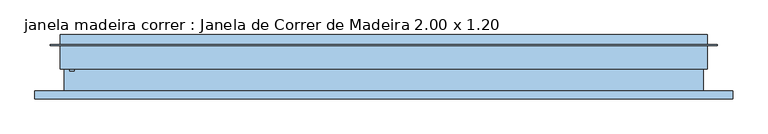
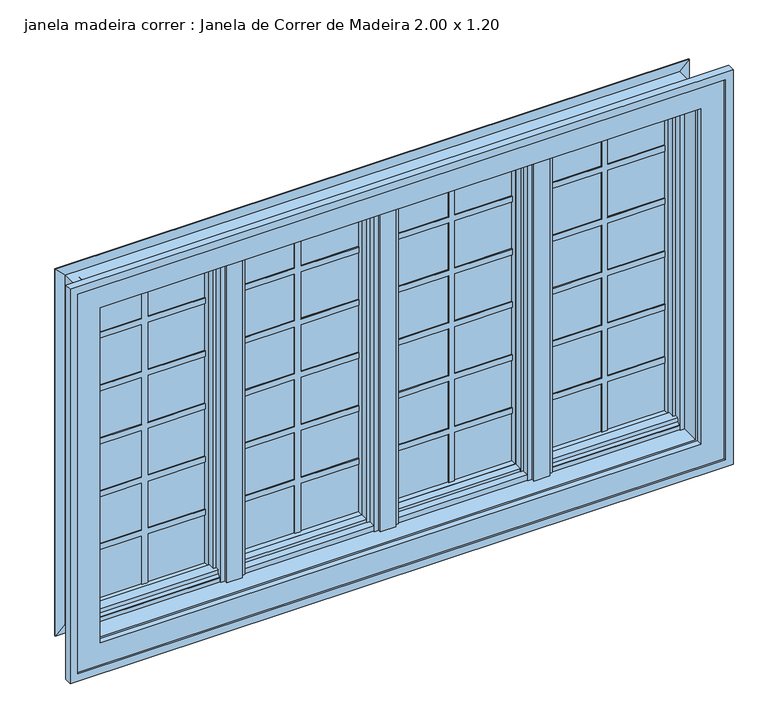
"""IFC4 building model written with IfcOpenShell, lengths in millimetres: window geometry, janela madeira correr : Janela de Correr de Madeira 2.00 x 1.20."""

import ifcopenshell
import ifcopenshell.guid

model = None  # the IFC model being written
_history = None  # IfcOwnerHistory: only IFC2X3 demands one
_inside = {}  # id of a spatial element -> (the spatial element, [elements in it])
_under = {}  # id of a project, library or spatial element -> (it, [spatial elements below it])
_declared = {}  # id of a project -> (the project, [libraries it declares])
_typed = {}  # id of a type object -> (the type object, [elements of that type])
_made_of = {}  # id of a material, layer set ... -> (it, [elements and type objects made of it])


def new_model(schema):
    """Start an empty IFC model of exactly this schema.

    Asked for "IFC4X3", IfcOpenShell would pick the latest addendum, in which some entities
    have other attributes; the version numbers below select the first issue.
    IFC2X3 requires an IfcOwnerHistory on every rooted entity: one is made here for all.
    """
    global model, _history
    if schema == "IFC4X3":
        model = ifcopenshell.file(schema_version=(4, 3, 0, 0))
    else:
        model = ifcopenshell.file(schema=schema)
    _inside.clear()
    _under.clear()
    _declared.clear()
    _typed.clear()
    _made_of.clear()
    _history = None
    if model.schema == "IFC2X3":
        org = make("IfcOrganization", Name="unknown")
        user = make(
            "IfcPersonAndOrganization",
            ThePerson=make("IfcPerson", FamilyName="unknown"),
            TheOrganization=org,
        )
        app = make(
            "IfcApplication",
            ApplicationDeveloper=org,
            Version="unknown",
            ApplicationFullName="unknown",
            ApplicationIdentifier="unknown",
        )
        _history = make(
            "IfcOwnerHistory",
            OwningUser=user,
            OwningApplication=app,
            ChangeAction="ADDED",
            CreationDate=0,
        )
    return model


def make(cls, **values):
    """One entity of the class cls with the attributes given. An attribute that is None is left unset."""
    return model.create_entity(
        cls, **{name: value for name, value in values.items() if value is not None}
    )


def rooted(cls, **values):
    """An entity with a GlobalId (a new one), such as an element, a storey or a relation."""
    return make(cls, GlobalId=ifcopenshell.guid.new(), OwnerHistory=_history, **values)


def si_unit(unit_type, name, prefix=None):
    """IfcSIUnit, for example si_unit("LENGTHUNIT", "METRE", prefix="MILLI")."""
    return make("IfcSIUnit", UnitType=unit_type, Prefix=prefix, Name=name)


def assignment(units):
    """IfcUnitAssignment: the units of a project."""
    return None if units is None else make("IfcUnitAssignment", Units=units)


def point(xyz):
    """IfcCartesianPoint."""
    return None if xyz is None else make("IfcCartesianPoint", Coordinates=xyz)


def direction(xyz):
    """IfcDirection."""
    return None if xyz is None else make("IfcDirection", DirectionRatios=xyz)


def frame(location, z_axis=None, x_axis=None):
    """IfcAxis2Placement3D, a coordinate frame: its origin and axes. An axis left out is left unset."""
    return make(
        "IfcAxis2Placement3D",
        Location=point(location),
        Axis=direction(z_axis),
        RefDirection=direction(x_axis),
    )


def origin():
    """The frame at (0, 0, 0) with its axes left unset."""
    return frame((0.0, 0.0, 0.0))


def place(relative_to, where):
    """IfcLocalPlacement: puts the frame where relative to a parent placement (None: the world)."""
    return make(
        "IfcLocalPlacement", PlacementRelTo=relative_to, RelativePlacement=where
    )


def context(
    kind, dimensions, precision=None, world=None, true_north=None, identifier=None
):
    """IfcGeometricRepresentationContext, for example the 3D "Model" context."""
    return make(
        "IfcGeometricRepresentationContext",
        ContextIdentifier=identifier,
        ContextType=kind,
        CoordinateSpaceDimension=dimensions,
        Precision=precision,
        WorldCoordinateSystem=world,
        TrueNorth=true_north,
    )


def project(units=None, contexts=None):
    """IfcProject with its units and contexts."""
    return rooted(
        "IfcProject",
        Name="project",
        RepresentationContexts=contexts,
        UnitsInContext=assignment(units),
    )


def spatial(cls, under=None, at=None, **own):
    """A site, building, storey or space (cls), placed at a placement, below another one or the project."""
    s = rooted(cls, ObjectPlacement=at, **own)
    if under is not None:
        _under.setdefault(under.id(), (under, []))[1].append(s)
    return s


def polyline(points):
    """IfcPolyline through the points."""
    return make("IfcPolyline", Points=[point(p) for p in points])


def outline(outer, holes=None, kind="AREA"):
    """IfcArbitraryClosedProfileDef: a profile drawn as a closed curve; with holes, ...WithVoids."""
    if holes is None:
        return make("IfcArbitraryClosedProfileDef", ProfileType=kind, OuterCurve=outer)
    return make(
        "IfcArbitraryProfileDefWithVoids",
        ProfileType=kind,
        OuterCurve=outer,
        InnerCurves=holes,
    )


def extrude(swept, where, along, depth):
    """IfcExtrudedAreaSolid: the profile swept, set in the frame where, extruded along a direction by depth."""
    return make(
        "IfcExtrudedAreaSolid",
        SweptArea=swept,
        Position=where,
        ExtrudedDirection=direction(along),
        Depth=depth,
    )


def faces_of(points, faces, orient=None, outer=None):
    """IfcFace entities. A face is a list of loops; a loop is a list of indices into points, from 0.

    orient and outer hold one flag for each loop. By default every Orientation is true, the
    first loop of a face is its IfcFaceOuterBound and the others are IfcFaceBound.
    """
    made = []
    for i, loops in enumerate(faces):
        bounds = []
        for j, loop in enumerate(loops):
            is_outer = j == 0 if outer is None else outer[i][j]
            bounds.append(
                make(
                    "IfcFaceOuterBound" if is_outer else "IfcFaceBound",
                    Bound=make("IfcPolyLoop", Polygon=[points[k] for k in loop]),
                    Orientation=True if orient is None else orient[i][j],
                )
            )
        made.append(make("IfcFace", Bounds=bounds))
    return made


def faceted_brep(points, faces, orient=None, outer=None, voids=None):
    """IfcFacetedBrep: a solid bounded by flat faces; with voids (closed shells), ...WithVoids."""
    shared = [point(p) for p in points]
    hull = make("IfcClosedShell", CfsFaces=faces_of(shared, faces, orient, outer))
    if voids is None:
        return make("IfcFacetedBrep", Outer=hull)
    return make(
        "IfcFacetedBrepWithVoids",
        Outer=hull,
        Voids=[
            make(cls, CfsFaces=faces_of(shared, fs, o, b)) for cls, fs, o, b in voids
        ],
    )


def shape(context_of_items, identifier, shape_type, items):
    """IfcShapeRepresentation: the items that make up one representation, for example the "Body"."""
    return make(
        "IfcShapeRepresentation",
        ContextOfItems=context_of_items,
        RepresentationIdentifier=identifier,
        RepresentationType=shape_type,
        Items=items,
    )


def source(mapping_origin, context_of_items, identifier, shape_type, items):
    """IfcRepresentationMap: a shape defined once, which mapped items show again and again."""
    return make(
        "IfcRepresentationMap",
        MappingOrigin=mapping_origin,
        MappedRepresentation=shape(context_of_items, identifier, shape_type, items),
    )


def transform(
    local_origin,
    x_axis=None,
    y_axis=None,
    z_axis=None,
    scale=None,
    scale2=None,
    scale3=None,
    uniform=True,
):
    """IfcCartesianTransformationOperator3D, or its non-uniform kind. x_axis, y_axis, z_axis: its Axis1, 2, 3."""
    if uniform:
        return make(
            "IfcCartesianTransformationOperator3D",
            Axis1=direction(x_axis),
            Axis2=direction(y_axis),
            LocalOrigin=point(local_origin),
            Scale=scale,
            Axis3=direction(z_axis),
        )
    return make(
        "IfcCartesianTransformationOperator3DnonUniform",
        Axis1=direction(x_axis),
        Axis2=direction(y_axis),
        LocalOrigin=point(local_origin),
        Scale=scale,
        Axis3=direction(z_axis),
        Scale2=scale2,
        Scale3=scale3,
    )


def mapped(mapping_source, mapping_target):
    """IfcMappedItem: shows the shape of a source again, moved by a transform."""
    return make(
        "IfcMappedItem", MappingSource=mapping_source, MappingTarget=mapping_target
    )


def made_of(thing, what):
    """Note that an element or type object is made of a material, layer set ...; save() writes the relation."""
    if what is not None:
        _made_of.setdefault(what.id(), (what, []))[1].append(thing)
    return thing


def element(
    cls,
    number,
    at=None,
    inside=None,
    cuts=None,
    type_object=None,
    material=None,
    context=None,
    identifier="Body",
    shape_type=None,
    held_by="IfcProductDefinitionShape",
    body=None,
    shapes=None,
    **own,
):
    """One element of the class cls, such as IfcWall. Its Tag is "e" and its number.

    at: its placement. inside: the storey or other place that contains it. cuts: it is an
    opening in that element (IfcRelVoidsElement). A single representation is given by context,
    identifier, shape_type and body (its items); several are given by shapes. held_by: the class
    of the entity that holds the representations. save() writes the other relations.
    """
    e = rooted(cls, Tag="e%d" % number, ObjectPlacement=at, **own)
    if body is not None:
        shapes = [shape(context, identifier, shape_type, body)]
    if shapes is not None:
        e.Representation = make(held_by, Representations=shapes)
    if inside is not None:
        _inside.setdefault(inside.id(), (inside, []))[1].append(e)
    if cuts is not None:
        rooted(
            "IfcRelVoidsElement", RelatingBuildingElement=cuts, RelatedOpeningElement=e
        )
    if type_object is not None:
        _typed.setdefault(type_object.id(), (type_object, []))[1].append(e)
    return made_of(e, material)


def aggregate(whole, parts):
    """IfcRelAggregates: a whole, such as a stair, and the parts it consists of."""
    return rooted("IfcRelAggregates", RelatingObject=whole, RelatedObjects=parts)


def save(model, path):
    """Write the relations noted so far, then the file.

    IfcRelAggregates (storeys below a building ...), IfcRelContainedInSpatialStructure (elements
    in a storey), IfcRelDefinesByType, IfcRelAssociatesMaterial and IfcRelDeclares: one each for
    every whole, place, type object, material and project.
    """
    for whole, parts in _under.values():
        aggregate(whole, parts)
    for where, things in _inside.values():
        rooted(
            "IfcRelContainedInSpatialStructure",
            RelatedElements=things,
            RelatingStructure=where,
        )
    for kind, things in _typed.values():
        rooted("IfcRelDefinesByType", RelatedObjects=things, RelatingType=kind)
    for what, things in _made_of.values():
        rooted("IfcRelAssociatesMaterial", RelatedObjects=things, RelatingMaterial=what)
    for by, libraries in _declared.values():
        rooted("IfcRelDeclares", RelatingContext=by, RelatedDefinitions=libraries)
    model.write(path)


def janela_madeira_correr_janela_de_correr_de_madeira_2_00_x_1_d447c460(model_context):
    return source(origin(), model_context, "Body", "SolidModel", [
        extrude(outline(polyline([(1881.6300584, 206.5264803), (1881.6300584, 13.2337398), (1862.5800584, 13.2337398), (1862.5800584, 206.5264803), (1699.6775292, 206.5264803), (1699.6775292, 13.2337398), (1680.6275292, 13.2337398), (1680.6275292, 206.5264803), (1517.725, 206.5264803), (1517.725, 13.2337398), (1498.675, 13.2337398), (1498.675, 206.5264803), (1335.7724708, 206.5264803), (1335.7724708, 13.2337398), (1316.7224708, 13.2337398), (1316.7224708, 206.5264803), (1153.8199416, 206.5264803), (1153.8199416, 13.2337398), (1134.7699416, 13.2337398), (1134.7699416, 206.5264803), (962.3424123, 206.5264803), (962.3424123, 225.5764803), (1134.7699416, 225.5764803), (1134.7699416, 418.8692207), (1153.8199416, 418.8692207), (1153.8199416, 225.5764803), (1316.7224708, 225.5764803), (1316.7224708, 418.8692207), (1335.7724708, 418.8692207), (1335.7724708, 225.5764803), (1498.675, 225.5764803), (1498.675, 418.8692207), (1517.725, 418.8692207), (1517.725, 225.5764803), (1680.6275292, 225.5764803), (1680.6275292, 418.8692207), (1699.6775292, 418.8692207), (1699.6775292, 225.5764803), (1862.5800584, 225.5764803), (1862.5800584, 418.8692207), (1881.6300584, 418.8692207), (1881.6300584, 225.5764803), (2054.0575877, 225.5764803), (2054.0575877, 206.5264803), (1881.6300584, 206.5264803)])), frame((0.0, 46.9582456, 0.0), z_axis=(0.0, 1.0, 0.0), x_axis=(0.0, 0.0, 1.0)), (0.0, 0.0, 1.0), 3.1432544),
        extrude(outline(polyline([(1881.6300584, -293.4735197), (1881.6300584, -486.7662602), (1862.5800584, -486.7662602), (1862.5800584, -293.4735197), (1699.6775292, -293.4735197), (1699.6775292, -486.7662602), (1680.6275292, -486.7662602), (1680.6275292, -293.4735197), (1517.725, -293.4735197), (1517.725, -486.7662602), (1498.675, -486.7662602), (1498.675, -293.4735197), (1335.7724708, -293.4735197), (1335.7724708, -486.7662602), (1316.7224708, -486.7662602), (1316.7224708, -293.4735197), (1153.8199416, -293.4735197), (1153.8199416, -486.7662602), (1134.7699416, -486.7662602), (1134.7699416, -293.4735197), (962.3424123, -293.4735197), (962.3424123, -274.4235197), (1134.7699416, -274.4235197), (1134.7699416, -81.1307793), (1153.8199416, -81.1307793), (1153.8199416, -274.4235197), (1316.7224708, -274.4235197), (1316.7224708, -81.1307793), (1335.7724708, -81.1307793), (1335.7724708, -274.4235197), (1498.675, -274.4235197), (1498.675, -81.1307793), (1517.725, -81.1307793), (1517.725, -274.4235197), (1680.6275292, -274.4235197), (1680.6275292, -81.1307793), (1699.6775292, -81.1307793), (1699.6775292, -274.4235197), (1862.5800584, -274.4235197), (1862.5800584, -81.1307793), (1881.6300584, -81.1307793), (1881.6300584, -274.4235197), (2054.0575877, -274.4235197), (2054.0575877, -293.4735197), (1881.6300584, -293.4735197)])), frame((0.0, 46.9582456, 0.0), z_axis=(0.0, 1.0, 0.0), x_axis=(0.0, 0.0, 1.0)), (0.0, 0.0, 1.0), 3.1432544),
        extrude(outline(polyline([(1881.6300584, 206.5264803), (1881.6300584, 13.2337398), (1862.5800584, 13.2337398), (1862.5800584, 206.5264803), (1699.6775292, 206.5264803), (1699.6775292, 13.2337398), (1680.6275292, 13.2337398), (1680.6275292, 206.5264803), (1517.725, 206.5264803), (1517.725, 13.2337398), (1498.675, 13.2337398), (1498.675, 206.5264803), (1335.7724708, 206.5264803), (1335.7724708, 13.2337398), (1316.7224708, 13.2337398), (1316.7224708, 206.5264803), (1153.6503822, 206.5264803), (1153.6503822, 13.2337398), (1134.6003822, 13.2337398), (1134.6003822, 206.5264803), (962.3424123, 206.5264803), (962.3424123, 225.5764803), (1134.6003822, 225.5764803), (1134.6003822, 418.8692207), (1153.6503822, 418.8692207), (1153.6503822, 225.5764803), (1316.7224708, 225.5764803), (1316.7224708, 418.8692207), (1335.7724708, 418.8692207), (1335.7724708, 225.5764803), (1498.675, 225.5764803), (1498.675, 418.8692207), (1517.725, 418.8692207), (1517.725, 225.5764803), (1680.6275292, 225.5764803), (1680.6275292, 418.8692207), (1699.6775292, 418.8692207), (1699.6775292, 225.5764803), (1862.5800584, 225.5764803), (1862.5800584, 418.8692207), (1881.6300584, 418.8692207), (1881.6300584, 225.5764803), (2054.0575877, 225.5764803), (2054.0575877, 206.5264803), (1881.6300584, 206.5264803)])), frame((0.0, 50.1015, 0.0), z_axis=(0.0, 1.0, 0.0), x_axis=(0.0, 0.0, 1.0)), (0.0, 0.0, 1.0), 15.875),
        extrude(outline(polyline([(1881.6300584, -293.4735197), (1881.6300584, -486.7662602), (1862.5800584, -486.7662602), (1862.5800584, -293.4735197), (1699.6775292, -293.4735197), (1699.6775292, -486.7662602), (1680.6275292, -486.7662602), (1680.6275292, -293.4735197), (1517.725, -293.4735197), (1517.725, -486.7662602), (1498.675, -486.7662602), (1498.675, -293.4735197), (1335.7724708, -293.4735197), (1335.7724708, -486.7662602), (1316.7224708, -486.7662602), (1316.7224708, -293.4735197), (1153.8199416, -293.4735197), (1153.8199416, -486.7662602), (1134.7699416, -486.7662602), (1134.7699416, -293.4735197), (962.3424123, -293.4735197), (962.3424123, -274.4235197), (1134.7699416, -274.4235197), (1134.7699416, -81.1307793), (1153.8199416, -81.1307793), (1153.8199416, -274.4235197), (1316.7224708, -274.4235197), (1316.7224708, -81.1307793), (1335.7724708, -81.1307793), (1335.7724708, -274.4235197), (1498.675, -274.4235197), (1498.675, -81.1307793), (1517.725, -81.1307793), (1517.725, -274.4235197), (1680.6275292, -274.4235197), (1680.6275292, -81.1307793), (1699.6775292, -81.1307793), (1699.6775292, -274.4235197), (1862.5800584, -274.4235197), (1862.5800584, -81.1307793), (1881.6300584, -81.1307793), (1881.6300584, -274.4235197), (2054.0575877, -274.4235197), (2054.0575877, -293.4735197), (1881.6300584, -293.4735197)])), frame((0.0, 50.1015, 0.0), z_axis=(0.0, 1.0, 0.0), x_axis=(0.0, 0.0, 1.0)), (0.0, 0.0, 1.0), 15.875),
        extrude(outline(polyline([(-79.1922697, 50.1015), (-488.7047697, 50.1015), (-488.7047697, 65.9765), (-79.1922697, 65.9765), (-79.1922697, 50.1015)])), frame((0.0, 0.0, 962.3424123), z_axis=(0.0, 0.0, 1.0), x_axis=(1.0, 0.0, 0.0)), (0.0, 0.0, 1.0), 1091.7151753),
        faceted_brep([(1019.5438803, -105.0, 855.00605), (1019.5438803, -98.65, 855.00605), (-1087.4409197, -98.65, 855.00605), (-1087.4409197, -105.0, 855.00605), (1044.9438803, -79.6, 829.60605), (1044.9438803, -105.0, 829.60605), (-1112.8409197, -105.0, 829.60605), (-1112.8409197, -79.6, 829.60605), (943.3438803, -98.65, 931.20605), (943.3438803, -79.6, 931.20605), (-1011.2409197, -79.6, 931.20605), (-1011.2409197, -98.65, 931.20605), (-1087.4409197, -98.65, 2161.72415), (-1087.4409197, -105.0, 2161.72415), (-1112.8409197, -105.0, 2187.12415), (-1112.8409197, -79.6, 2187.12415), (-1011.2409197, -79.6, 2085.52415), (-1011.2409197, -98.65, 2085.52415), (1019.5438803, -98.65, 2161.72415), (1019.5438803, -105.0, 2161.72415), (1044.9438803, -105.0, 2187.12415), (1044.9438803, -79.6, 2187.12415), (943.3438803, -79.6, 2085.52415), (943.3438803, -98.65, 2085.52415)], [[[0, 1, 2, 3]], [[4, 5, 6, 7]], [[8, 9, 10, 11]], [[3, 2, 12, 13]], [[7, 6, 14, 15]], [[11, 10, 16, 17]], [[13, 12, 18, 19]], [[15, 14, 20, 21]], [[17, 16, 22, 23]], [[1, 18, 12, 2], [11, 17, 23, 8]], [[19, 18, 1, 0]], [[5, 20, 14, 6], [3, 13, 19, 0]], [[21, 20, 5, 4]], [[7, 15, 21, 4], [9, 22, 16, 10]], [[23, 22, 9, 8]]]),
        extrude(outline(polyline([(1153.8199416, 723.716552), (1316.7224708, 723.716552), (1316.7224708, 917.0878737), (1335.7724708, 917.0878737), (1335.7724708, 723.716552), (1498.675, 723.716552), (1498.675, 917.0878737), (1517.725, 917.0878737), (1517.725, 723.716552), (1680.6275292, 723.716552), (1680.6275292, 917.0878737), (1699.6775292, 917.0878737), (1699.6775292, 723.716552), (1862.5800584, 723.716552), (1862.5800584, 917.0878737), (1881.6300584, 917.0878737), (1881.6300584, 723.716552), (2054.0575877, 723.716552), (2054.0575877, 704.666552), (1881.6300584, 704.666552), (1881.6300584, 511.2952303), (1862.5800584, 511.2952303), (1862.5800584, 704.666552), (1699.6775292, 704.666552), (1699.6775292, 511.2952303), (1680.6275292, 511.2952303), (1680.6275292, 704.666552), (1517.725, 704.666552), (1517.725, 511.2952303), (1498.675, 511.2952303), (1498.675, 704.666552), (1335.7724708, 704.666552), (1335.7724708, 511.2952303), (1316.7224708, 511.2952303), (1316.7224708, 704.666552), (1153.8199416, 704.666552), (1153.8199416, 511.2952303), (1134.7699416, 511.2952303), (1134.7699416, 704.666552), (962.3424123, 704.666552), (962.3424123, 723.716552), (1134.7699416, 723.716552), (1134.7699416, 917.0878737), (1153.8199416, 917.0878737), (1153.8199416, 723.716552)])), frame((0.0, 46.7303732, 0.0), z_axis=(0.0, 1.0, 0.0), x_axis=(0.0, 0.0, 1.0)), (0.0, 0.0, 1.0), 3.3711268),
        extrude(outline(polyline([(1881.6300584, -791.6417168), (1881.6300584, -984.9344572), (1862.5800584, -984.9344572), (1862.5800584, -791.6417168), (1699.6775292, -791.6417168), (1699.6775292, -984.9344572), (1680.6275292, -984.9344572), (1680.6275292, -791.6417168), (1517.725, -791.6417168), (1517.725, -984.9344572), (1498.675, -984.9344572), (1498.675, -791.6417168), (1335.7724708, -791.6417168), (1335.7724708, -984.9344572), (1316.7224708, -984.9344572), (1316.7224708, -791.6417168), (1153.8199416, -791.6417168), (1153.8199416, -984.9344572), (1134.7699416, -984.9344572), (1134.7699416, -791.6417168), (962.3424123, -791.6417168), (962.3424123, -772.5917168), (1134.7699416, -772.5917168), (1134.7699416, -579.2989763), (1153.8199416, -579.2989763), (1153.8199416, -772.5917168), (1316.7224708, -772.5917168), (1316.7224708, -579.2989763), (1335.7724708, -579.2989763), (1335.7724708, -772.5917168), (1498.675, -772.5917168), (1498.675, -579.2989763), (1517.725, -579.2989763), (1517.725, -772.5917168), (1680.6275292, -772.5917168), (1680.6275292, -579.2989763), (1699.6775292, -579.2989763), (1699.6775292, -772.5917168), (1862.5800584, -772.5917168), (1862.5800584, -579.2989763), (1881.6300584, -579.2989763), (1881.6300584, -772.5917168), (2054.0575877, -772.5917168), (2054.0575877, -791.6417168), (1881.6300584, -791.6417168)])), frame((0.0, 46.9582456, 0.0), z_axis=(0.0, 1.0, 0.0), x_axis=(0.0, 0.0, 1.0)), (0.0, 0.0, 1.0), 3.1432544),
        extrude(outline(polyline([(35.1373, 2049.7546), (9.8065079, 2049.7546), (9.2928, 2058.8986), (-15.6627, 2058.8986), (-15.6627, 2079.17415), (-11.7892, 2079.17415), (-11.7892, 2072.0304), (35.1373, 2072.0304), (35.1373, 2049.7546)])), frame((-494.6547197, 0.0, 0.0), z_axis=(1.0, 0.0, 0.0), x_axis=(0.0, 1.0, 0.0)), (0.0, 0.0, 1.0), 921.4124),
        extrude(outline(polyline([(35.1373, 965.477), (35.1373, 944.3696), (-11.7892, 944.3696), (-11.7892, 937.55605), (-15.6627, 937.55605), (-15.6627, 955.952), (9.0471115, 955.952), (9.8065079, 965.477), (35.1373, 965.477)])), frame((-494.6547197, 0.0, 0.0), z_axis=(1.0, 0.0, 0.0), x_axis=(0.0, 1.0, 0.0)), (0.0, 0.0, 1.0), 921.4124),
        extrude(outline(polyline([(35.1373, 2049.7546), (9.8065079, 2049.7546), (9.2928, 2058.8986), (-15.6627, 2058.8986), (-15.6627, 2079.17415), (-11.7892, 2079.17415), (-11.7892, 2072.0304), (35.1373, 2072.0304), (35.1373, 2049.7546)])), frame((-990.9971197, 0.0, 0.0), z_axis=(1.0, 0.0, 0.0), x_axis=(0.0, 1.0, 0.0)), (0.0, 0.0, 1.0), 417.6462326),
        extrude(outline(polyline([(35.1373, 965.477), (35.1373, 944.3696), (-11.7892, 944.3696), (-11.7892, 937.55605), (-15.6627, 937.55605), (-15.6627, 951.5578), (-12.2972, 951.5578), (-5.0582, 959.4826), (-3.9768196, 973.0462), (27.9364, 973.0462), (35.1373, 965.477)])), frame((-990.9971197, 0.0, 0.0), z_axis=(1.0, 0.0, 0.0), x_axis=(0.0, 1.0, 0.0)), (0.0, 0.0, 1.0), 417.6462326),
        faceted_brep([(454.9389803, 85.9373, 2088.2955442), (454.9389803, 48.6374, 2088.2955442), (454.9389803, 48.6374, 2069.8909496), (454.9389803, 35.1373, 2067.5291599), (454.9389803, 35.1373, 2050.1057516), (454.9389803, 48.6374, 2047.8865571), (454.9389803, 48.6374, 968.5290777), (454.9389803, 35.1373, 966.3098832), (454.9389803, 35.1373, 948.8864749), (454.9389803, 48.6374, 946.5246852), (454.9389803, 48.6374, 928.1044558), (454.9389803, 85.9373, 928.1044558), (-23.7161471, 85.9373, 2088.2955442), (-23.7161471, 85.9373, 2059.2701124), (-23.7161471, 74.7560374, 2057.8452835), (-23.7161471, 74.4029109, 2047.2338554), (-23.7161471, 69.3765, 2044.5482224), (-23.7161471, 69.3765, 2060.523579), (-23.7161471, 53.5015, 2060.523579), (-23.7161471, 53.5015, 2047.086979), (-23.7161471, 35.1373, 2050.1057516), (-23.7161471, 35.1373, 2067.5291599), (-23.7161471, 48.6374, 2069.8909496), (-23.7161471, 48.6374, 2088.2955442), (-23.7161471, 53.5015, 969.3286558), (-23.7161471, 53.5015, 955.8920558), (-23.7161471, 69.3765, 955.8920558), (-23.7161471, 69.3765, 971.8674123), (-23.7161471, 74.4029109, 969.1817794), (-23.7161471, 74.7560374, 958.5703513), (-23.7161471, 85.9373, 957.1455224), (-23.7161471, 85.9373, 928.1044558), (-23.7161471, 48.6374, 928.1044558), (-23.7161471, 48.6374, 946.5246852), (-23.7161471, 35.1373, 948.8864749), (-23.7161471, 35.1373, 966.3098832), (-4.4157903, 48.6374, 2088.2955442), (-2.0540006, 35.1373, 2088.2955442), (15.3694077, 35.1373, 2088.2955442), (17.5886022, 48.6374, 2088.2955442), (414.5143584, 48.6374, 2088.2955442), (416.7335529, 35.1373, 2088.2955442), (434.1569612, 35.1373, 2088.2955442), (436.5187509, 48.6374, 2088.2955442), (436.5187509, 48.6374, 2069.8909496), (-22.8360197, 48.6374, 2069.8909496), (-4.4157903, 48.6374, 2069.8909496), (17.5886022, 48.6374, 2069.8909496), (414.5143584, 48.6374, 2069.8909496), (434.1569612, 35.1373, 2067.5291599), (-2.0540006, 35.1373, 2067.5291599), (15.3694077, 35.1373, 2067.5291599), (416.7335529, 35.1373, 2067.5291599), (-2.0540006, 35.1373, 928.1044558), (15.3694077, 35.1373, 928.1044558), (15.3694077, 35.1373, 948.8864749), (416.7335529, 35.1373, 948.8864749), (416.7335529, 35.1373, 928.1044558), (434.1569612, 35.1373, 928.1044558), (434.1569612, 35.1373, 948.8864749), (434.1569612, 35.1373, 966.3098832), (434.1569612, 35.1373, 2050.1057516), (-2.0540006, 35.1373, 2050.1057516), (-2.0540006, 35.1373, 966.3098832), (-2.0540006, 35.1373, 948.8864749), (416.7335529, 35.1373, 2050.1057516), (416.7335529, 35.1373, 966.3098832), (15.3694077, 35.1373, 966.3098832), (15.3694077, 35.1373, 2050.1057516), (436.5187509, 48.6374, 2047.8865571), (-22.8360197, 53.5015, 2047.086979), (-22.8360197, 48.6374, 2047.8865571), (-4.4157903, 48.6374, 2047.8865571), (18.3881803, 53.5015, 2047.086979), (413.7147803, 53.5015, 2047.086979), (-22.8360197, 53.5015, 2060.523579), (-22.8360197, 53.5015, 969.3286558), (-22.8360197, 53.5015, 955.8920558), (427.1513803, 53.5015, 2060.523579), (427.1513803, 53.5015, 955.8920558), (4.9515803, 53.5015, 955.8920558), (4.9515803, 53.5015, 2060.523579), (18.3881803, 53.5015, 969.3286558), (413.7147803, 53.5015, 969.3286558), (-22.8360197, 69.3765, 2060.523579), (4.9515803, 69.3765, 2060.523579), (427.1513803, 69.3765, 2060.523579), (-22.8360197, 69.3765, 2044.5482224), (-22.8360197, 69.3765, 955.8920558), (-22.8360197, 69.3765, 971.8674123), (4.9515803, 69.3765, 955.8920558), (427.1513803, 69.3765, 955.8920558), (411.1760237, 69.3765, 2044.5482224), (411.1760237, 69.3765, 971.8674123), (20.9269368, 69.3765, 971.8674123), (20.9269368, 69.3765, 2044.5482224), (-22.8360197, 74.4029109, 2047.2338554), (18.2413039, 74.4029109, 2047.2338554), (413.8616566, 74.4029109, 2047.2338554), (-22.8360197, 74.7560374, 2057.8452835), (7.6298758, 74.7560374, 2057.8452835), (424.4730847, 74.7560374, 2057.8452835), (-22.8360197, 85.9373, 2059.2701124), (6.2050469, 85.9373, 2059.2701124), (425.8979136, 85.9373, 2059.2701124), (-22.8360197, 85.9373, 957.1455224), (6.2050469, 85.9373, 957.1455224), (425.8979136, 85.9373, 957.1455224), (436.5187509, 48.6374, 968.5290777), (-4.4157903, 48.6374, 968.5290777), (-22.8360197, 48.6374, 968.5290777), (436.5187509, 48.6374, 946.5246852), (-22.8360197, 48.6374, 946.5246852), (-4.4157903, 48.6374, 946.5246852), (17.5886022, 48.6374, 946.5246852), (414.5143584, 48.6374, 946.5246852), (436.5187509, 48.6374, 928.1044558), (-4.4157903, 48.6374, 928.1044558), (17.5886022, 48.6374, 928.1044558), (414.5143584, 48.6374, 928.1044558), (-22.8360197, 74.7560374, 958.5703513), (7.6298758, 74.7560374, 958.5703513), (424.4730847, 74.7560374, 958.5703513), (-22.8360197, 74.4029109, 969.1817794), (18.2413039, 74.4029109, 969.1817794), (413.8616566, 74.4029109, 969.1817794)], [[[0, 1, 2, 3, 4, 5, 6, 7, 8, 9, 10, 11]], [[12, 13, 14, 15, 16, 17, 18, 19, 20, 21, 22, 23]], [[24, 25, 26, 27, 28, 29, 30, 31, 32, 33, 34, 35]], [[1, 0, 12, 23, 36, 37, 38, 39, 40, 41, 42, 43]], [[2, 1, 43, 44]], [[36, 23, 22, 45, 46]], [[40, 39, 47, 48]], [[3, 2, 44, 49]], [[22, 21, 50, 46, 45]], [[48, 47, 51, 52]], [[53, 54, 55, 56, 57, 58, 59, 8, 7, 60, 61, 4, 3, 49, 42, 41, 52, 51, 38, 37, 50, 21, 20, 62, 63, 35, 34, 64], [65, 66, 67, 68]], [[5, 4, 61, 69]], [[20, 19, 70, 71, 72, 62]], [[65, 68, 73, 74]], [[19, 18, 75, 70]], [[25, 24, 76, 77]], [[78, 79, 80, 81], [74, 73, 82, 83]], [[18, 17, 84, 75]], [[78, 81, 85, 86]], [[17, 16, 87, 84]], [[27, 26, 88, 89]], [[86, 85, 90, 91], [92, 93, 94, 95]], [[16, 15, 96, 87]], [[92, 95, 97, 98]], [[15, 14, 99, 96]], [[98, 97, 100, 101]], [[14, 13, 102, 99]], [[101, 100, 103, 104]], [[12, 0, 11, 31, 30, 105, 102, 13], [103, 106, 107, 104]], [[7, 6, 108, 60]], [[24, 35, 63, 109, 110, 76]], [[83, 82, 67, 66]], [[9, 8, 59, 111]], [[34, 33, 112, 113, 64]], [[56, 55, 114, 115]], [[10, 9, 111, 116]], [[33, 32, 117, 113, 112]], [[115, 114, 118, 119]], [[31, 11, 10, 116, 58, 57, 119, 118, 54, 53, 117, 32]], [[30, 29, 120, 105]], [[107, 106, 121, 122]], [[29, 28, 123, 120]], [[122, 121, 124, 125]], [[28, 27, 89, 123]], [[125, 124, 94, 93]], [[26, 25, 77, 88]], [[91, 90, 80, 79]], [[101, 122, 125, 98]], [[104, 107, 122, 101]], [[6, 5, 69, 108]], [[43, 42, 49, 44]], [[61, 60, 108, 69]], [[58, 116, 111, 59]], [[41, 40, 48, 52]], [[57, 56, 115, 119]], [[74, 83, 66, 65]], [[79, 78, 86, 91]], [[98, 125, 93, 92]], [[124, 97, 95, 94]], [[81, 80, 90, 85]], [[39, 38, 51, 47]], [[55, 54, 118, 114]], [[82, 73, 68, 67]], [[37, 36, 46, 50]], [[63, 62, 72, 109]], [[117, 53, 64, 113]], [[109, 72, 71, 110]], [[102, 105, 120, 123, 89, 88, 77, 76, 110, 71, 70, 75, 84, 87, 96, 99]], [[106, 103, 100, 121]], [[121, 100, 97, 124]]]),
        faceted_brep([(-86.1383434, 74.4029109, 2088.2955442), (-88.8239763, 69.3765, 2088.2955442), (-72.8486197, 69.3765, 2088.2955442), (-72.8486197, 53.5015, 2088.2955442), (-86.2852197, 53.5015, 2088.2955442), (-83.2664471, 35.1373, 2088.2955442), (-65.8430388, 35.1373, 2088.2955442), (-63.4812491, 48.6374, 2088.2955442), (-45.0610197, 48.6374, 2088.2955442), (-45.0610197, 85.9373, 2088.2955442), (-74.1020864, 85.9373, 2088.2955442), (-75.5269153, 74.7560374, 2088.2955442), (-86.1383434, 74.4029109, 928.1044558), (-75.5269153, 74.7560374, 928.1044558), (-74.1020864, 85.9373, 928.1044558), (-45.0610197, 85.9373, 928.1044558), (-45.0610197, 48.6374, 928.1044558), (-63.4812491, 48.6374, 928.1044558), (-65.8430388, 35.1373, 928.1044558), (-83.2664471, 35.1373, 928.1044558), (-86.2852197, 53.5015, 928.1044558), (-72.8486197, 53.5015, 928.1044558), (-72.8486197, 69.3765, 928.1044558), (-88.8239763, 69.3765, 928.1044558)], [[[0, 1, 2, 3, 4, 5, 6, 7, 8, 9, 10, 11]], [[12, 13, 14, 15, 16, 17, 18, 19, 20, 21, 22, 23]], [[13, 12, 0, 11]], [[14, 13, 11, 10]], [[15, 14, 10, 9]], [[16, 15, 9, 8]], [[17, 16, 8, 7]], [[18, 17, 7, 6]], [[19, 18, 6, 5]], [[20, 19, 5, 4]], [[21, 20, 4, 3]], [[22, 21, 3, 2]], [[23, 22, 2, 1]], [[12, 23, 1, 0]]]),
        faceted_brep([(-481.7586961, 74.4029109, 2088.2955442), (-492.3701242, 74.7560374, 2088.2955442), (-493.7949531, 85.9373, 2088.2955442), (-522.8360197, 85.9373, 2088.2955442), (-522.8360197, 48.6374, 2088.2955442), (-504.4157903, 48.6374, 2088.2955442), (-502.0540006, 35.1373, 2088.2955442), (-484.6305923, 35.1373, 2088.2955442), (-481.6118197, 53.5015, 2088.2955442), (-495.0484197, 53.5015, 2088.2955442), (-495.0484197, 69.3765, 2088.2955442), (-479.0730632, 69.3765, 2088.2955442), (-481.7586961, 74.4029109, 928.1044558), (-479.0730632, 69.3765, 928.1044558), (-495.0484197, 69.3765, 928.1044558), (-495.0484197, 53.5015, 928.1044558), (-481.6118197, 53.5015, 928.1044558), (-484.6305923, 35.1373, 928.1044558), (-502.0540006, 35.1373, 928.1044558), (-504.4157903, 48.6374, 928.1044558), (-522.8360197, 48.6374, 928.1044558), (-522.8360197, 85.9373, 928.1044558), (-493.7949531, 85.9373, 928.1044558), (-492.3701242, 74.7560374, 928.1044558)], [[[0, 1, 2, 3, 4, 5, 6, 7, 8, 9, 10, 11]], [[12, 13, 14, 15, 16, 17, 18, 19, 20, 21, 22, 23]], [[13, 12, 0, 11]], [[14, 13, 11, 10]], [[15, 14, 10, 9]], [[16, 15, 9, 8]], [[17, 16, 8, 7]], [[18, 17, 7, 6]], [[19, 18, 6, 5]], [[20, 19, 5, 4]], [[21, 20, 4, 3]], [[22, 21, 3, 2]], [[23, 22, 2, 1]], [[12, 23, 1, 0]]]),
        extrude(outline(polyline([(35.1373, 2049.7546), (9.8065079, 2049.7546), (9.2928, 2058.8986), (-15.6627, 2058.8986), (-15.6627, 2079.17415), (-11.7892, 2079.17415), (-11.7892, 2072.0304), (35.1373, 2072.0304), (35.1373, 2049.7546)])), frame((502.0932267, 0.0, 0.0), z_axis=(1.0, 0.0, 0.0), x_axis=(0.0, 1.0, 0.0)), (0.0, 0.0, 1.0), 424.1385817),
        extrude(outline(polyline([(35.1373, 965.477), (35.1373, 944.3696), (-11.7892, 944.3696), (-11.7892, 937.55605), (-15.6627, 937.55605), (-15.6627, 951.5578), (-12.2972, 951.5578), (-5.0582, 959.4826), (-3.9768196, 973.0462), (27.9364, 973.0462), (35.1373, 965.477)])), frame((502.0932267, 0.0, 0.0), z_axis=(1.0, 0.0, 0.0), x_axis=(0.0, 1.0, 0.0)), (0.0, 0.0, 1.0), 424.1385817),
        extrude(outline(polyline([(-59.3485197, 32.1945), (-59.3485197, -19.05), (-73.2423197, -19.05), (-73.2423197, 6.35), (-82.3863197, 6.8637079), (-82.3863197, 32.1945), (-59.3485197, 32.1945)])), frame((0.0, 0.0, 937.55605), z_axis=(0.0, 0.0, 1.0), x_axis=(1.0, 0.0, 0.0)), (0.0, 0.0, 1.0), 1141.6181),
        extrude(outline(polyline([(-8.5485197, 32.1945), (14.4892803, 32.1945), (14.4892803, 6.8637079), (5.3452803, 6.35), (5.3452803, -19.05), (-8.5485197, -19.05), (-8.5485197, 32.1945)])), frame((0.0, 0.0, 937.55605), z_axis=(0.0, 0.0, 1.0), x_axis=(1.0, 0.0, 0.0)), (0.0, 0.0, 1.0), 1141.6181),
        extrude(outline(polyline([(420.8077303, 50.1015), (11.2952303, 50.1015), (11.2952303, 65.9765), (420.8077303, 65.9765), (420.8077303, 50.1015)])), frame((0.0, 0.0, 962.3424123), z_axis=(0.0, 0.0, 1.0), x_axis=(1.0, 0.0, 0.0)), (0.0, 0.0, 1.0), 1091.7151753),
        extrude(outline(polyline([(1153.8199416, 723.716552), (1316.7224708, 723.716552), (1316.7224708, 917.0878737), (1335.7724708, 917.0878737), (1335.7724708, 723.716552), (1498.675, 723.716552), (1498.675, 917.0878737), (1517.725, 917.0878737), (1517.725, 723.716552), (1680.6275292, 723.716552), (1680.6275292, 917.0878737), (1699.6775292, 917.0878737), (1699.6775292, 723.716552), (1862.5800584, 723.716552), (1862.5800584, 917.0878737), (1881.6300584, 917.0878737), (1881.6300584, 723.716552), (2054.0575877, 723.716552), (2054.0575877, 704.666552), (1881.6300584, 704.666552), (1881.6300584, 511.2952303), (1862.5800584, 511.2952303), (1862.5800584, 704.666552), (1699.6775292, 704.666552), (1699.6775292, 511.2952303), (1680.6275292, 511.2952303), (1680.6275292, 704.666552), (1517.725, 704.666552), (1517.725, 511.2952303), (1498.675, 511.2952303), (1498.675, 704.666552), (1335.7724708, 704.666552), (1335.7724708, 511.2952303), (1316.7224708, 511.2952303), (1316.7224708, 704.666552), (1153.8199416, 704.666552), (1153.8199416, 511.2952303), (1134.7699416, 511.2952303), (1134.7699416, 704.666552), (962.3424123, 704.666552), (962.3424123, 723.716552), (1134.7699416, 723.716552), (1134.7699416, 917.0878737), (1153.8199416, 917.0878737), (1153.8199416, 723.716552)])), frame((0.0, 50.1015, 0.0), z_axis=(0.0, 1.0, 0.0), x_axis=(0.0, 0.0, 1.0)), (0.0, 0.0, 1.0), 15.875),
        extrude(outline(polyline([(917.0878737, 50.1015), (511.2952303, 50.1015), (511.2952303, 65.9765), (917.0878737, 65.9765), (917.0878737, 50.1015)])), frame((0.0, 0.0, 962.3424123), z_axis=(0.0, 0.0, 1.0), x_axis=(1.0, 0.0, 0.0)), (0.0, 0.0, 1.0), 1091.8825877),
        extrude(outline(polyline([(440.6514803, -3.9768196), (440.6514803, 48.6374), (455.8191077, 48.6374), (459.7768673, 93.8748), (472.3260932, 93.8748), (476.2838529, 48.6374), (491.4514803, 48.6374), (491.4514803, -3.9768196), (440.6514803, -3.9768196)])), frame((0.0, 0.0, 925.6747737), z_axis=(0.0, 0.0, 1.0), x_axis=(1.0, 0.0, 0.0)), (0.0, 0.0, 1.0), 1165.0504526),
        extrude(outline(polyline([(-559.3485197, -3.9768196), (-559.3485197, 48.6374), (-544.1808923, 48.6374), (-540.2231327, 93.8748), (-527.6739068, 93.8748), (-523.7161471, 48.6374), (-508.5485197, 48.6374), (-508.5485197, -3.9768196), (-559.3485197, -3.9768196)])), frame((0.0, 0.0, 925.6747737), z_axis=(0.0, 0.0, 1.0), x_axis=(1.0, 0.0, 0.0)), (0.0, 0.0, 1.0), 1165.0504526),
        extrude(outline(polyline([(-59.3485197, -3.9768196), (-59.3485197, 48.6374), (-44.1808923, 48.6374), (-40.2231327, 93.8748), (-27.6739068, 93.8748), (-23.7161471, 48.6374), (-8.5485197, 48.6374), (-8.5485197, -3.9768196), (-59.3485197, -3.9768196)])), frame((0.0, 0.0, 925.6747737), z_axis=(0.0, 0.0, 1.0), x_axis=(1.0, 0.0, 0.0)), (0.0, 0.0, 1.0), 1165.0504526),
        faceted_brep([(951.3258303, 85.9373, 928.1044558), (951.3258303, 48.6374, 928.1044558), (932.9056009, 48.6374, 928.1044558), (930.5438112, 35.1373, 928.1044558), (913.1204029, 35.1373, 928.1044558), (910.9012084, 48.6374, 928.1044558), (517.5886022, 48.6374, 928.1044558), (515.3694077, 35.1373, 928.1044558), (497.9459994, 35.1373, 928.1044558), (495.5842097, 48.6374, 928.1044558), (477.1639803, 48.6374, 928.1044558), (477.1639803, 85.9373, 928.1044558), (913.1204029, 35.1373, 2079.6498291), (930.5438112, 35.1373, 2079.6498291), (932.9056009, 48.6374, 2079.6498291), (910.9012084, 48.6374, 2079.6498291), (495.5842097, 48.6374, 2079.6498291), (497.9459994, 35.1373, 2079.6498291), (515.3694077, 35.1373, 2079.6498291), (517.5886022, 48.6374, 2079.6498291), (910.2485066, 74.4029109, 969.1817794), (910.2485066, 74.4029109, 2047.2338554), (920.8599347, 74.7560374, 2057.8452835), (920.8599347, 74.7560374, 958.5703513), (922.2847636, 85.9373, 2059.2701124), (922.2847636, 85.9373, 957.1455224), (477.1639803, 85.9373, 2088.2955442), (951.3258303, 85.9373, 2088.2955442), (506.2050469, 85.9373, 2059.2701124), (506.2050469, 85.9373, 957.1455224), (951.3258303, 48.6374, 2088.2955442), (951.3258303, 48.6374, 2069.8909496), (951.3258303, 35.1373, 2067.5291599), (951.3258303, 35.1373, 2050.1057516), (951.3258303, 48.6374, 2047.8865571), (951.3258303, 48.6374, 968.5290777), (951.3258303, 35.1373, 966.3098832), (951.3258303, 35.1373, 948.8864749), (951.3258303, 48.6374, 946.5246852), (932.9056009, 48.6374, 946.5246852), (495.5842097, 48.6374, 946.5246852), (477.1639803, 48.6374, 946.5246852), (477.1639803, 48.6374, 2088.2955442), (477.1639803, 48.6374, 2069.8909496), (495.5842097, 48.6374, 2069.8909496), (517.5886022, 48.6374, 2069.8909496), (910.9012084, 48.6374, 2069.8909496), (932.9056009, 48.6374, 2069.8909496), (932.9056009, 48.6374, 2047.8865571), (932.9056009, 48.6374, 968.5290777), (495.5842097, 48.6374, 968.5290777), (495.5842097, 48.6374, 2047.8865571), (477.1639803, 48.6374, 2047.8865571), (477.1639803, 48.6374, 968.5290777), (930.5438112, 35.1373, 948.8864749), (930.5438112, 35.1373, 2067.5291599), (930.5438112, 35.1373, 2050.1057516), (930.5438112, 35.1373, 966.3098832), (477.1639803, 35.1373, 966.3098832), (477.1639803, 35.1373, 948.8864749), (497.9459994, 35.1373, 948.8864749), (515.3694077, 35.1373, 948.8864749), (913.1204029, 35.1373, 948.8864749), (913.1204029, 35.1373, 2067.5291599), (515.3694077, 35.1373, 2067.5291599), (497.9459994, 35.1373, 2067.5291599), (477.1639803, 35.1373, 2067.5291599), (477.1639803, 35.1373, 2050.1057516), (497.9459994, 35.1373, 2050.1057516), (497.9459994, 35.1373, 966.3098832), (913.1204029, 35.1373, 966.3098832), (515.3694077, 35.1373, 966.3098832), (515.3694077, 35.1373, 2050.1057516), (913.1204029, 35.1373, 2050.1057516), (910.9012084, 48.6374, 946.5246852), (910.1016303, 53.5015, 2047.086979), (910.1016303, 53.5015, 969.3286558), (923.5382303, 53.5015, 955.8920558), (504.9515803, 53.5015, 955.8920558), (504.9515803, 53.5015, 2060.523579), (923.5382303, 53.5015, 2060.523579), (518.3881803, 53.5015, 2047.086979), (518.3881803, 53.5015, 969.3286558), (923.5382303, 69.3765, 2060.523579), (923.5382303, 69.3765, 955.8920558), (504.9515803, 69.3765, 2060.523579), (504.9515803, 69.3765, 955.8920558), (907.5628737, 69.3765, 971.8674123), (520.9269368, 69.3765, 971.8674123), (520.9269368, 69.3765, 2044.5482224), (907.5628737, 69.3765, 2044.5482224), (518.2413039, 74.4029109, 969.1817794), (518.2413039, 74.4029109, 2047.2338554), (517.5886022, 48.6374, 946.5246852), (507.6298758, 74.7560374, 2057.8452835), (507.6298758, 74.7560374, 958.5703513)], [[[0, 1, 2, 3, 4, 5, 6, 7, 8, 9, 10, 11]], [[12, 13, 14, 15]], [[16, 17, 18, 19]], [[20, 21, 22, 23]], [[23, 22, 24, 25]], [[0, 11, 26, 27], [24, 28, 29, 25]], [[1, 0, 27, 30, 31, 32, 33, 34, 35, 36, 37, 38]], [[2, 1, 38, 39]], [[10, 9, 40, 41]], [[31, 30, 42, 43, 44, 16, 19, 45, 46, 15, 14, 47]], [[35, 34, 48, 49]], [[50, 51, 52, 53]], [[3, 2, 39, 54]], [[14, 13, 55, 47]], [[49, 48, 56, 57]], [[58, 59, 60, 8, 7, 61, 62, 4, 3, 54, 37, 36, 57, 56, 33, 32, 55, 13, 12, 63, 64, 18, 17, 65, 66, 67, 68, 69], [70, 71, 72, 73]], [[5, 4, 62, 74]], [[12, 15, 46, 63]], [[70, 73, 75, 76]], [[77, 78, 79, 80], [76, 75, 81, 82]], [[77, 80, 83, 84]], [[84, 83, 85, 86], [87, 88, 89, 90]], [[21, 20, 87, 90]], [[91, 92, 89, 88]], [[86, 85, 79, 78]], [[7, 6, 93, 61]], [[19, 18, 64, 45]], [[82, 81, 72, 71]], [[9, 8, 60, 40]], [[17, 16, 44, 65]], [[69, 68, 51, 50]], [[26, 11, 10, 41, 59, 58, 53, 52, 67, 66, 43, 42]], [[29, 28, 94, 95]], [[92, 91, 95, 94]], [[30, 27, 26, 42]], [[32, 31, 47, 55]], [[64, 63, 46, 45]], [[43, 66, 65, 44]], [[34, 33, 56, 48]], [[68, 67, 52, 51]], [[81, 75, 73, 72]], [[85, 83, 80, 79]], [[92, 21, 90, 89]], [[21, 92, 94, 22]], [[28, 24, 22, 94]], [[36, 35, 49, 57]], [[58, 69, 50, 53]], [[76, 82, 71, 70]], [[38, 37, 54, 39]], [[62, 61, 93, 74]], [[59, 41, 40, 60]], [[6, 5, 74, 93]], [[25, 29, 95, 23]], [[91, 20, 23, 95]], [[20, 91, 88, 87]], [[84, 86, 78, 77]]]),
        extrude(outline(polyline([(-559.3485197, -28.8072), (-559.3485197, -3.9768196), (-508.5485197, -3.9768196), (-508.5485197, -28.8072), (-559.3485197, -28.8072)])), frame((0.0, 0.0, 937.55605), z_axis=(0.0, 0.0, 1.0), x_axis=(1.0, 0.0, 0.0)), (0.0, 0.0, 1.0), 1141.6181),
        extrude(outline(polyline([(491.4514803, -28.8072), (440.6514803, -28.8072), (440.6514803, -3.9768196), (491.4514803, -3.9768196), (491.4514803, -28.8072)])), frame((0.0, 0.0, 937.55605), z_axis=(0.0, 0.0, 1.0), x_axis=(1.0, 0.0, 0.0)), (0.0, 0.0, 1.0), 1141.6181),
        extrude(outline(polyline([(-8.5485197, -28.8072), (-59.3485197, -28.8072), (-59.3485197, -3.9768196), (-8.5485197, -3.9768196), (-8.5485197, -28.8072)])), frame((0.0, 0.0, 937.55605), z_axis=(0.0, 0.0, 1.0), x_axis=(1.0, 0.0, 0.0)), (0.0, 0.0, 1.0), 1141.6181),
        extrude(outline(polyline([(-579.2989763, 50.1015), (-984.9344572, 50.1015), (-984.9344572, 65.9765), (-579.2989763, 65.9765), (-579.2989763, 50.1015)])), frame((0.0, 0.0, 962.3424123), z_axis=(0.0, 0.0, 1.0), x_axis=(1.0, 0.0, 0.0)), (0.0, 0.0, 1.0), 1091.8825877),
        extrude(outline(polyline([(1881.6300584, -791.6417168), (1881.6300584, -984.9344572), (1862.5800584, -984.9344572), (1862.5800584, -791.6417168), (1699.6775292, -791.6417168), (1699.6775292, -984.9344572), (1680.6275292, -984.9344572), (1680.6275292, -791.6417168), (1517.725, -791.6417168), (1517.725, -984.9344572), (1498.675, -984.9344572), (1498.675, -791.6417168), (1335.7724708, -791.6417168), (1335.7724708, -984.9344572), (1316.7224708, -984.9344572), (1316.7224708, -791.6417168), (1153.8199416, -791.6417168), (1153.8199416, -984.9344572), (1134.7699416, -984.9344572), (1134.7699416, -791.6417168), (962.3424123, -791.6417168), (962.3424123, -772.5917168), (1134.7699416, -772.5917168), (1134.7699416, -579.2989763), (1153.8199416, -579.2989763), (1153.8199416, -772.5917168), (1316.7224708, -772.5917168), (1316.7224708, -579.2989763), (1335.7724708, -579.2989763), (1335.7724708, -772.5917168), (1498.675, -772.5917168), (1498.675, -579.2989763), (1517.725, -579.2989763), (1517.725, -772.5917168), (1680.6275292, -772.5917168), (1680.6275292, -579.2989763), (1699.6775292, -579.2989763), (1699.6775292, -772.5917168), (1862.5800584, -772.5917168), (1862.5800584, -579.2989763), (1881.6300584, -579.2989763), (1881.6300584, -772.5917168), (2054.0575877, -772.5917168), (2054.0575877, -791.6417168), (1881.6300584, -791.6417168)])), frame((0.0, 50.1015, 0.0), z_axis=(0.0, 1.0, 0.0), x_axis=(0.0, 0.0, 1.0)), (0.0, 0.0, 1.0), 15.875),
        faceted_brep([(966.0514803, -11.7892, 908.2), (966.0514803, 93.8748, 908.2), (966.0514803, 93.8748, 2108.2), (966.0514803, -11.7892, 2108.2), (-1033.9485197, -11.7892, 2108.2), (-1033.9485197, 93.8748, 2108.2), (-1033.9485197, 93.8748, 908.2), (-1033.9485197, -11.7892, 908.2), (936.9938803, -11.7892, 2072.0304), (936.9938803, -11.7892, 944.3696), (-1004.8909197, -11.7892, 944.3696), (-1004.8909197, -11.7892, 2072.0304), (-1004.8909197, 48.6374, 2072.0304), (936.9938803, 48.6374, 2072.0304), (953.7070803, 48.6374, 2090.7252263), (953.7070803, 48.6374, 925.6747737), (-1021.6041197, 48.6374, 925.6747737), (-1021.6041197, 48.6374, 2090.7252263), (-1004.8909197, 48.6374, 944.3696), (936.9938803, 48.6374, 944.3696), (-1021.6041197, 93.8748, 2090.7252263), (953.7070803, 93.8748, 2090.7252263), (-1021.6041197, 93.8748, 925.6747737), (953.7070803, 93.8748, 925.6747737)], [[[0, 1, 2, 3]], [[4, 5, 6, 7]], [[0, 3, 4, 7], [8, 9, 10, 11]], [[8, 11, 12, 13]], [[14, 15, 16, 17], [13, 12, 18, 19]], [[14, 17, 20, 21]], [[2, 1, 6, 5], [20, 22, 23, 21]], [[4, 3, 2, 5]], [[23, 22, 16, 15]], [[19, 18, 10, 9]], [[6, 1, 0, 7]], [[13, 19, 9, 8]], [[21, 23, 15, 14]], [[22, 20, 17, 16]], [[18, 12, 11, 10]]]),
        extrude(outline(polyline([(920.10625, 954.4436803), (2096.62395, 954.4436803), (2096.62395, -1022.3407197), (920.10625, -1022.3407197), (920.10625, 954.4436803)]), holes=[polyline([(2079.17415, 936.9938803), (937.55605, 936.9938803), (937.55605, -1004.8909197), (2079.17415, -1004.8909197), (2079.17415, 936.9938803)])]), frame((0.0, -79.6, 0.0), z_axis=(0.0, 1.0, 0.0), x_axis=(0.0, 0.0, 1.0)), (0.0, 0.0, 1.0), 67.8108),
        faceted_brep([(-551.4110197, 48.6374, 2069.8753148), (-551.4110197, 35.1373, 2067.5135251), (-551.4110197, 35.1373, 2050.0901168), (-551.4110197, 48.6374, 2047.3667015), (-551.4110197, 35.1373, 965.589539), (-551.4110197, 35.1373, 948.8864749), (-551.4110197, 48.6374, 946.5246852), (-551.4110197, 48.6374, 967.8087335), (-1019.2228697, 85.9373, 928.1044558), (-1019.2228697, 48.6374, 928.1044558), (-1019.2228697, 48.6374, 946.5246852), (-1019.2228697, 35.1373, 948.8864749), (-1019.2228697, 35.1373, 965.589539), (-1019.2228697, 48.6374, 967.8087335), (-1019.2228697, 48.6374, 2047.3667015), (-1019.2228697, 35.1373, 2050.0901168), (-1019.2228697, 35.1373, 2067.5135251), (-1019.2228697, 48.6374, 2069.8753148), (-1019.2228697, 48.6374, 2088.2955442), (-1019.2228697, 85.9373, 2088.2955442), (-1000.8026403, 48.6374, 2088.2955442), (-998.4408506, 35.1373, 2088.2955442), (-981.0174423, 35.1373, 2088.2955442), (-978.7982478, 48.6374, 2088.2955442), (-585.4856416, 48.6374, 2088.2955442), (-583.2664471, 35.1373, 2088.2955442), (-565.8430388, 35.1373, 2088.2955442), (-563.4812491, 48.6374, 2088.2955442), (-545.0610197, 48.6374, 2088.2955442), (-545.0610197, 85.9373, 2088.2955442), (-1000.8026403, 48.6374, 928.1044558), (-1000.8026403, 48.6374, 946.5246852), (-1000.8026403, 48.6374, 2069.8753148), (-978.7982478, 48.6374, 2069.8753148), (-585.4856416, 48.6374, 2069.8753148), (-563.4812491, 48.6374, 2069.8753148), (-563.4812491, 48.6374, 2047.3667015), (-563.4812491, 48.6374, 967.8087335), (-563.4812491, 48.6374, 946.5246852), (-563.4812491, 48.6374, 928.1044558), (-545.0610197, 48.6374, 928.1044558), (-585.4856416, 48.6374, 946.5246852), (-978.7982478, 48.6374, 946.5246852), (-978.7982478, 48.6374, 928.1044558), (-585.4856416, 48.6374, 928.1044558), (-565.8430388, 35.1373, 2067.5135251), (-998.4408506, 35.1373, 2067.5135251), (-981.0174423, 35.1373, 2067.5135251), (-583.2664471, 35.1373, 2067.5135251), (-583.2664471, 35.1373, 928.1044558), (-565.8430388, 35.1373, 928.1044558), (-565.8430388, 35.1373, 948.8864749), (-565.8430388, 35.1373, 965.589539), (-565.8430388, 35.1373, 2050.0901168), (-998.4408506, 35.1373, 2050.0901168), (-998.4408506, 35.1373, 965.589539), (-998.4408506, 35.1373, 948.8864749), (-998.4408506, 35.1373, 928.1044558), (-981.0174423, 35.1373, 928.1044558), (-981.0174423, 35.1373, 948.8864749), (-583.2664471, 35.1373, 948.8864749), (-583.2664471, 35.1373, 2050.0901168), (-583.2664471, 35.1373, 965.589539), (-981.0174423, 35.1373, 965.589539), (-981.0174423, 35.1373, 2050.0901168), (-1000.8026403, 48.6374, 2047.3667015), (-978.5575738, 50.1015, 2047.0713442), (-585.7263156, 50.1015, 2047.0713442), (-978.5575738, 50.1015, 2060.5079442), (-585.7263156, 50.1015, 2060.5079442), (-977.9986697, 53.5015, 2060.5079442), (-991.4352697, 53.5015, 2060.5079442), (-991.4352697, 65.9765, 2060.5079442), (-572.8486197, 65.9765, 2060.5079442), (-572.8486197, 53.5015, 2060.5079442), (-586.2852197, 53.5015, 2060.5079442), (-991.4352697, 65.9765, 2044.5325877), (-572.8486197, 65.9765, 2044.5325877), (-991.4352697, 69.3765, 2046.3492223), (-975.4599132, 69.3765, 2046.3492223), (-976.3289115, 71.0029109, 2047.2182206), (-587.954978, 71.0029109, 2047.2182206), (-588.8239763, 69.3765, 2046.3492223), (-572.8486197, 69.3765, 2046.3492223), (-976.5175885, 71.3560374, 2057.8296487), (-587.7663009, 71.3560374, 2057.8296487), (-978.1455461, 74.4029109, 2058.1273783), (-988.7569742, 74.7560374, 2058.1618845), (-990.1818031, 85.9373, 2059.2544776), (-574.1020864, 85.9373, 2059.2544776), (-575.5269153, 74.7560374, 2058.1618845), (-586.1383434, 74.4029109, 2058.1273783), (-545.0610197, 85.9373, 928.1044558), (-990.1818031, 85.9373, 957.1455224), (-574.1020864, 85.9373, 957.1455224), (-1000.8026403, 48.6374, 967.8087335), (-586.2852197, 53.5015, 968.6083116), (-977.9986697, 53.5015, 968.6083116), (-988.7569742, 74.7560374, 958.5703513), (-575.5269153, 74.7560374, 958.5703513), (-978.1455461, 74.4029109, 969.1817794), (-586.1383434, 74.4029109, 969.1817794), (-975.4599132, 69.3765, 971.8674123), (-588.8239763, 69.3765, 971.8674123), (-572.8486197, 69.3765, 955.8920558), (-991.4352697, 69.3765, 955.8920558), (-991.4352697, 53.5015, 955.8920558), (-572.8486197, 53.5015, 955.8920558)], [[[0, 1, 2, 3]], [[4, 5, 6, 7]], [[8, 9, 10, 11, 12, 13, 14, 15, 16, 17, 18, 19]], [[19, 18, 20, 21, 22, 23, 24, 25, 26, 27, 28, 29]], [[10, 9, 30, 31]], [[18, 17, 32, 20]], [[24, 23, 33, 34]], [[28, 27, 35, 0, 3, 36, 37, 7, 6, 38, 39, 40]], [[41, 42, 43, 44]], [[1, 0, 35, 45]], [[17, 16, 46, 32]], [[34, 33, 47, 48]], [[49, 50, 51, 5, 4, 52, 53, 2, 1, 45, 26, 25, 48, 47, 22, 21, 46, 16, 15, 54, 55, 12, 11, 56, 57, 58, 59, 60], [61, 62, 63, 64]], [[3, 2, 53, 36]], [[15, 14, 65, 54]], [[61, 64, 66, 67]], [[67, 66, 68, 69]], [[69, 68, 70, 71, 72, 73, 74, 75]], [[73, 72, 76, 77]], [[77, 76, 78, 79, 80, 81, 82, 83]], [[81, 80, 84, 85]], [[85, 84, 86, 87, 88, 89, 90, 91]], [[8, 19, 29, 92], [88, 93, 94, 89]], [[4, 7, 37, 52]], [[13, 12, 55, 95]], [[96, 97, 63, 62]], [[6, 5, 51, 38]], [[11, 10, 31, 56]], [[60, 59, 42, 41]], [[9, 8, 92, 40, 39, 50, 49, 44, 43, 58, 57, 30]], [[94, 93, 98, 99]], [[99, 98, 100, 101]], [[101, 100, 102, 103]], [[104, 105, 106, 107]], [[100, 86, 84, 80, 79, 102]], [[105, 78, 76, 72, 71, 106]], [[23, 22, 47, 33]], [[64, 63, 97, 70, 68, 66]], [[59, 58, 43, 42]], [[21, 20, 32, 46]], [[55, 54, 65, 95]], [[30, 57, 56, 31]], [[14, 13, 95, 65]], [[93, 88, 87, 98]], [[86, 100, 98, 87]], [[101, 91, 90, 99]], [[89, 94, 99, 90]], [[40, 92, 29, 28]], [[27, 26, 45, 35]], [[53, 52, 37, 36]], [[50, 39, 38, 51]], [[25, 24, 34, 48]], [[62, 61, 67, 69, 75, 96]], [[49, 60, 41, 44]], [[107, 74, 73, 77, 83, 104]], [[91, 101, 103, 82, 81, 85]], [[103, 102, 79, 78, 105, 104, 83, 82]], [[97, 96, 75, 74, 107, 106, 71, 70]]]),
        faceted_brep([(-1033.9485197, 63.725, 908.2), (-1065.6985197, 63.725, 876.45), (-1065.6985197, 63.725, 2139.95), (-1033.9485197, 63.725, 2108.2), (-1033.9485197, 60.55, 908.2), (-1033.9485197, 60.55, 2108.2), (-1065.6985197, 60.55, 876.45), (-1065.6985197, 60.55, 2139.95), (997.8014803, 63.725, 2139.95), (966.0514803, 63.725, 2108.2), (966.0514803, 60.55, 2108.2), (997.8014803, 60.55, 2139.95), (997.8014803, 63.725, 876.45), (966.0514803, 63.725, 908.2), (966.0514803, 60.55, 908.2), (997.8014803, 60.55, 876.45)], [[[0, 1, 2, 3]], [[4, 0, 3, 5]], [[6, 4, 5, 7]], [[1, 6, 7, 2]], [[3, 2, 8, 9]], [[5, 3, 9, 10]], [[7, 5, 10, 11]], [[2, 7, 11, 8]], [[9, 8, 12, 13]], [[10, 9, 13, 14]], [[11, 10, 14, 15]], [[8, 11, 15, 12]], [[13, 12, 1, 0]], [[14, 13, 0, 4]], [[15, 14, 4, 6]], [[12, 15, 6, 1]]]),
        extrude(outline(polyline([(50.1015, 969.3286558), (50.1015, 955.8920558), (65.9765, 955.8920558), (65.9765, 971.8674123), (71.0029109, 969.1817794), (71.3560374, 958.5703513), (85.9373, 957.1455224), (85.9373, 928.1044558), (45.2374, 928.1044558), (45.2374, 946.5246852), (35.1373, 948.8864749), (35.1373, 966.3098832), (50.1015, 969.3286558)])), frame((-523.7161471, 0.0, 0.0), z_axis=(1.0, 0.0, 0.0), x_axis=(0.0, 1.0, 0.0)), (0.0, 0.0, 1.0), 479.5352548),
        extrude(outline(polyline([(85.9373, 2088.2955442), (85.9373, 2059.2701124), (71.3560374, 2057.8452835), (71.0029109, 2047.2338554), (65.9765, 2044.5482224), (65.9765, 2060.523579), (50.1015, 2060.523579), (50.1015, 2047.086979), (35.1373, 2050.1057516), (35.1373, 2067.5291599), (45.2374, 2069.8909496), (45.2374, 2088.2955442), (85.9373, 2088.2955442)])), frame((-523.7161471, 0.0, 0.0), z_axis=(1.0, 0.0, 0.0), x_axis=(0.0, 1.0, 0.0)), (0.0, 0.0, 1.0), 479.5352548),
        extrude(outline(polyline([(-1004.5797697, 32.1945), (-981.5419697, 32.1945), (-981.5419697, 6.8637079), (-990.6859697, 6.35), (-990.6859697, -19.05), (-1004.5797697, -19.05), (-1004.5797697, 32.1945)])), frame((0.0, 0.0, 908.2), z_axis=(0.0, 0.0, 1.0), x_axis=(1.0, 0.0, 0.0)), (0.0, 0.0, 1.0), 1200.0),
        extrude(outline(polyline([(936.6827303, 32.1945), (936.6827303, -19.05), (922.7889303, -19.05), (922.7889303, 6.35), (913.6449303, 6.8637079), (913.6449303, 32.1945), (936.6827303, 32.1945)])), frame((0.0, 0.0, 937.55605), z_axis=(0.0, 0.0, 1.0), x_axis=(1.0, 0.0, 0.0)), (0.0, 0.0, 1.0), 1141.6181),
        extrude(outline(polyline([(491.4514803, 32.1945), (514.4892803, 32.1945), (514.4892803, 6.8637079), (505.3452803, 6.35), (505.3452803, -19.05), (491.4514803, -19.05), (491.4514803, 32.1945)])), frame((0.0, 0.0, 937.55605), z_axis=(0.0, 0.0, 1.0), x_axis=(1.0, 0.0, 0.0)), (0.0, 0.0, 1.0), 1141.6181),
        extrude(outline(polyline([(440.6514803, 32.1945), (440.6514803, -19.05), (426.7576803, -19.05), (426.7576803, 6.35), (417.6136803, 6.8637079), (417.6136803, 32.1945), (440.6514803, 32.1945)])), frame((0.0, 0.0, 937.55605), z_axis=(0.0, 0.0, 1.0), x_axis=(1.0, 0.0, 0.0)), (0.0, 0.0, 1.0), 1141.6181),
        extrude(outline(polyline([(-559.3485197, 32.1945), (-559.3485197, -19.05), (-573.2423197, -19.05), (-573.2423197, 6.35), (-582.3863197, 6.8637079), (-582.3863197, 32.1945), (-559.3485197, 32.1945)])), frame((0.0, 0.0, 937.55605), z_axis=(0.0, 0.0, 1.0), x_axis=(1.0, 0.0, 0.0)), (0.0, 0.0, 1.0), 1141.6181),
        extrude(outline(polyline([(-508.5485197, 32.1945), (-485.5107197, 32.1945), (-485.5107197, 6.8637079), (-494.6547197, 6.35), (-494.6547197, -19.05), (-508.5485197, -19.05), (-508.5485197, 32.1945)])), frame((0.0, 0.0, 937.55605), z_axis=(0.0, 0.0, 1.0), x_axis=(1.0, 0.0, 0.0)), (0.0, 0.0, 1.0), 1141.6181),
    ])


if __name__ == "__main__":
    model = new_model("IFC4")
    model_context = context("Model", 3, world=origin())
    ifc_project = project(units=[si_unit("LENGTHUNIT", "METRE", prefix="MILLI")], contexts=[model_context])
    site = spatial("IfcSite", under=ifc_project)
    building = spatial("IfcBuilding", under=site)
    placement = place(None, origin())
    janela_madeira_correr_janela_de_correr_de_madeira_2_00_x_1_shape = janela_madeira_correr_janela_de_correr_de_madeira_2_00_x_1_d447c460(model_context)
    element("IfcWindow", 1, ObjectType="janela madeira correr : Janela de Correr de Madeira 2.00 x 1.20", at=placement, inside=building, context=model_context, shape_type="MappedRepresentation", body=[
        mapped(janela_madeira_correr_janela_de_correr_de_madeira_2_00_x_1_shape, transform((0.0, 0.0, 0.0), x_axis=(1.0, 0.0, 0.0), y_axis=(0.0, 1.0, 0.0), z_axis=(0.0, 0.0, 1.0))),
    ])
    save(model, "model.ifc")

# Revit data of these elements
# Type "janela madeira correr : Janela de Correr de Madeira 2.00 x 1.20"
#   Type Mark = "J11"
#   Analytic Construction = "<Nenhum>"
#   Description = "400 Series Casement - Triple Sash"
#   Manufacturer = "Andersen Corporation"
#   Construction Type = "Vinyl Clad Wood"
#   Model = "CW26-2"
#   Type Comments = "Shown w/ Optional Extension Jamb"
#   Rough Width = 2.00 m
#   Rough Height = 1.20 m
#   Default Sill Height = 0.9082 m
#   Default Head Height = 2.1082 m
#   Height = 1.20 m
#   Installation Flange Inset [instance default] = 0.01905 m
#   Width = 2.00 m
#   Wall Closure = (empty or 0)
# Element 1 (IfcWindow, "janela madeira correr : Janela de Correr de Madeira 2.00 x 1.20")
#   Materials on its faces: "Andersen(R) - White", "Andersen(R) - Pine Interior", "Vidro"
# Materials
#   "Andersen(R) - White": class "Não atribuído", colour RGB 249 249 249, transparency 0
#   "Andersen(R) - Pine Interior": class "Não atribuído", colour RGB 212 179 113, transparency 0
#   "Vidro": class "Vidro", colour RGB 0 128 192, transparency 0.9, Description = "Vidro de sílica", Cost = 0
